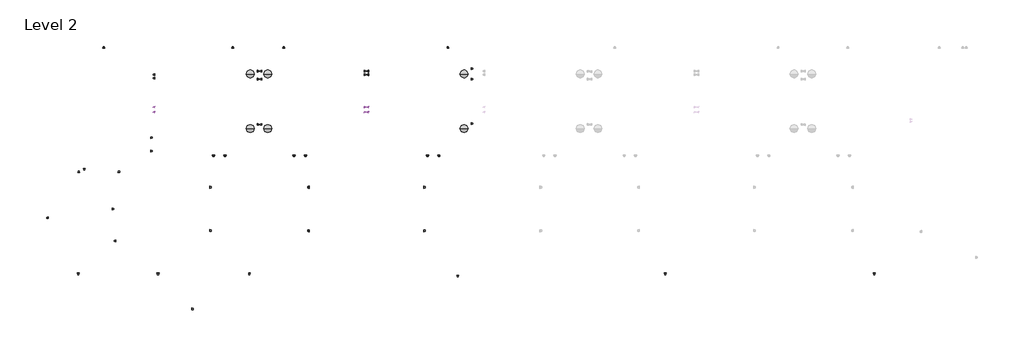
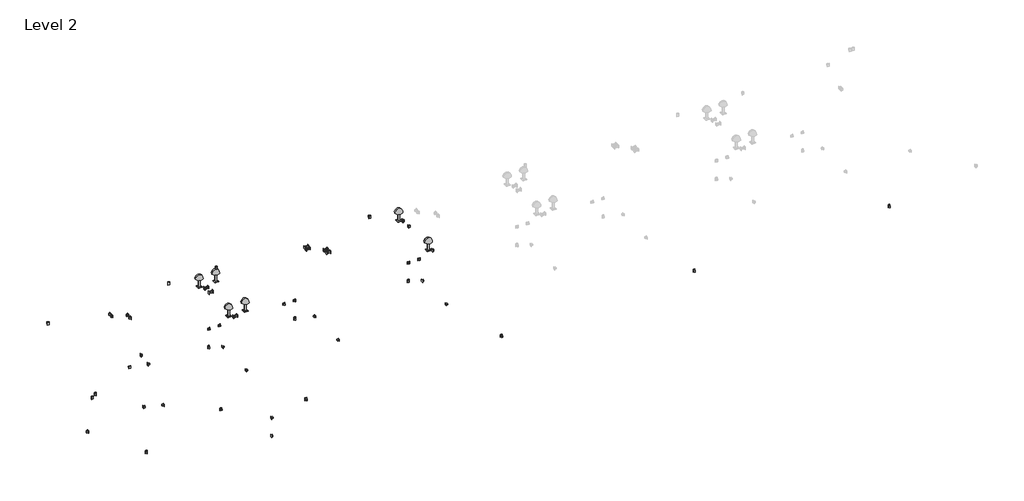
# One storey, part 1 of 2: 40 proxies, 16 switching devices, 6 light fixtures.
"""IFC4 building model written with IfcOpenShell, lengths in millimetres."""

import ifcopenshell
import ifcopenshell.guid

model = None  # the IFC model being written
_history = None  # IfcOwnerHistory: only IFC2X3 demands one
_inside = {}  # id of a spatial element -> (the spatial element, [elements in it])
_under = {}  # id of a project, library or spatial element -> (it, [spatial elements below it])
_declared = {}  # id of a project -> (the project, [libraries it declares])
_typed = {}  # id of a type object -> (the type object, [elements of that type])
_made_of = {}  # id of a material, layer set ... -> (it, [elements and type objects made of it])


def new_model(schema):
    """Start an empty IFC model of exactly this schema.

    Asked for "IFC4X3", IfcOpenShell would pick the latest addendum, in which some entities
    have other attributes; the version numbers below select the first issue.
    IFC2X3 requires an IfcOwnerHistory on every rooted entity: one is made here for all.
    """
    global model, _history
    if schema == "IFC4X3":
        model = ifcopenshell.file(schema_version=(4, 3, 0, 0))
    else:
        model = ifcopenshell.file(schema=schema)
    _inside.clear()
    _under.clear()
    _declared.clear()
    _typed.clear()
    _made_of.clear()
    _history = None
    if model.schema == "IFC2X3":
        org = make("IfcOrganization", Name="unknown")
        user = make(
            "IfcPersonAndOrganization",
            ThePerson=make("IfcPerson", FamilyName="unknown"),
            TheOrganization=org,
        )
        app = make(
            "IfcApplication",
            ApplicationDeveloper=org,
            Version="unknown",
            ApplicationFullName="unknown",
            ApplicationIdentifier="unknown",
        )
        _history = make(
            "IfcOwnerHistory",
            OwningUser=user,
            OwningApplication=app,
            ChangeAction="ADDED",
            CreationDate=0,
        )
    return model


def make(cls, **values):
    """One entity of the class cls with the attributes given. An attribute that is None is left unset."""
    return model.create_entity(
        cls, **{name: value for name, value in values.items() if value is not None}
    )


def rooted(cls, **values):
    """An entity with a GlobalId (a new one), such as an element, a storey or a relation."""
    return make(cls, GlobalId=ifcopenshell.guid.new(), OwnerHistory=_history, **values)


def si_unit(unit_type, name, prefix=None):
    """IfcSIUnit, for example si_unit("LENGTHUNIT", "METRE", prefix="MILLI")."""
    return make("IfcSIUnit", UnitType=unit_type, Prefix=prefix, Name=name)


def assignment(units):
    """IfcUnitAssignment: the units of a project."""
    return None if units is None else make("IfcUnitAssignment", Units=units)


def point(xyz):
    """IfcCartesianPoint."""
    return None if xyz is None else make("IfcCartesianPoint", Coordinates=xyz)


def direction(xyz):
    """IfcDirection."""
    return None if xyz is None else make("IfcDirection", DirectionRatios=xyz)


def frame(location, z_axis=None, x_axis=None):
    """IfcAxis2Placement3D, a coordinate frame: its origin and axes. An axis left out is left unset."""
    return make(
        "IfcAxis2Placement3D",
        Location=point(location),
        Axis=direction(z_axis),
        RefDirection=direction(x_axis),
    )


def frame_2d(location, x_axis=None):
    """IfcAxis2Placement2D, a coordinate frame in the plane: its origin and x axis."""
    return make(
        "IfcAxis2Placement2D", Location=point(location), RefDirection=direction(x_axis)
    )


def origin():
    """The frame at (0, 0, 0) with its axes left unset."""
    return frame((0.0, 0.0, 0.0))


def origin_with_axes():
    """The frame at (0, 0, 0) with the z axis (0, 0, 1) and the x axis (1, 0, 0) written out."""
    return frame((0.0, 0.0, 0.0), z_axis=(0.0, 0.0, 1.0), x_axis=(1.0, 0.0, 0.0))


def origin_2d():
    """The frame at (0, 0) in the plane with its x axis left unset."""
    return frame_2d((0.0, 0.0))


def place(relative_to, where):
    """IfcLocalPlacement: puts the frame where relative to a parent placement (None: the world)."""
    return make(
        "IfcLocalPlacement", PlacementRelTo=relative_to, RelativePlacement=where
    )


def context(
    kind, dimensions, precision=None, world=None, true_north=None, identifier=None
):
    """IfcGeometricRepresentationContext, for example the 3D "Model" context."""
    return make(
        "IfcGeometricRepresentationContext",
        ContextIdentifier=identifier,
        ContextType=kind,
        CoordinateSpaceDimension=dimensions,
        Precision=precision,
        WorldCoordinateSystem=world,
        TrueNorth=true_north,
    )


def project(units=None, contexts=None):
    """IfcProject with its units and contexts."""
    return rooted(
        "IfcProject",
        Name="project",
        RepresentationContexts=contexts,
        UnitsInContext=assignment(units),
    )


def spatial(cls, under=None, at=None, **own):
    """A site, building, storey or space (cls), placed at a placement, below another one or the project."""
    s = rooted(cls, ObjectPlacement=at, **own)
    if under is not None:
        _under.setdefault(under.id(), (under, []))[1].append(s)
    return s


def polyline(points):
    """IfcPolyline through the points."""
    return make("IfcPolyline", Points=[point(p) for p in points])


def circle_curve(where, radius):
    """IfcCircle in the frame where."""
    return make("IfcCircle", Position=where, Radius=radius)


def ellipse_curve(where, semi_axis1, semi_axis2):
    """IfcEllipse in the frame where."""
    return make(
        "IfcEllipse", Position=where, SemiAxis1=semi_axis1, SemiAxis2=semi_axis2
    )


def trimmed(basis, trim1, trim2, sense, master):
    """IfcTrimmedCurve: the piece of a basis curve between two trims."""
    return make(
        "IfcTrimmedCurve",
        BasisCurve=basis,
        Trim1=trim1,
        Trim2=trim2,
        SenseAgreement=sense,
        MasterRepresentation=master,
    )


def segment(curve, same_sense, transition):
    """IfcCompositeCurveSegment."""
    return make(
        "IfcCompositeCurveSegment",
        Transition=transition,
        SameSense=same_sense,
        ParentCurve=curve,
    )


def composite_curve(segments, self_intersect=None):
    """IfcCompositeCurve: segments joined end to end."""
    return make("IfcCompositeCurve", Segments=segments, SelfIntersect=self_intersect)


def outline(outer, holes=None, kind="AREA"):
    """IfcArbitraryClosedProfileDef: a profile drawn as a closed curve; with holes, ...WithVoids."""
    if holes is None:
        return make("IfcArbitraryClosedProfileDef", ProfileType=kind, OuterCurve=outer)
    return make(
        "IfcArbitraryProfileDefWithVoids",
        ProfileType=kind,
        OuterCurve=outer,
        InnerCurves=holes,
    )


def extrude(swept, where, along, depth):
    """IfcExtrudedAreaSolid: the profile swept, set in the frame where, extruded along a direction by depth."""
    return make(
        "IfcExtrudedAreaSolid",
        SweptArea=swept,
        Position=where,
        ExtrudedDirection=direction(along),
        Depth=depth,
    )


def shape(context_of_items, identifier, shape_type, items):
    """IfcShapeRepresentation: the items that make up one representation, for example the "Body"."""
    return make(
        "IfcShapeRepresentation",
        ContextOfItems=context_of_items,
        RepresentationIdentifier=identifier,
        RepresentationType=shape_type,
        Items=items,
    )


def source(mapping_origin, context_of_items, identifier, shape_type, items):
    """IfcRepresentationMap: a shape defined once, which mapped items show again and again."""
    return make(
        "IfcRepresentationMap",
        MappingOrigin=mapping_origin,
        MappedRepresentation=shape(context_of_items, identifier, shape_type, items),
    )


def transform(
    local_origin,
    x_axis=None,
    y_axis=None,
    z_axis=None,
    scale=None,
    scale2=None,
    scale3=None,
    uniform=True,
):
    """IfcCartesianTransformationOperator3D, or its non-uniform kind. x_axis, y_axis, z_axis: its Axis1, 2, 3."""
    if uniform:
        return make(
            "IfcCartesianTransformationOperator3D",
            Axis1=direction(x_axis),
            Axis2=direction(y_axis),
            LocalOrigin=point(local_origin),
            Scale=scale,
            Axis3=direction(z_axis),
        )
    return make(
        "IfcCartesianTransformationOperator3DnonUniform",
        Axis1=direction(x_axis),
        Axis2=direction(y_axis),
        LocalOrigin=point(local_origin),
        Scale=scale,
        Axis3=direction(z_axis),
        Scale2=scale2,
        Scale3=scale3,
    )


def mapped(mapping_source, mapping_target):
    """IfcMappedItem: shows the shape of a source again, moved by a transform."""
    return make(
        "IfcMappedItem", MappingSource=mapping_source, MappingTarget=mapping_target
    )


def made_of(thing, what):
    """Note that an element or type object is made of a material, layer set ...; save() writes the relation."""
    if what is not None:
        _made_of.setdefault(what.id(), (what, []))[1].append(thing)
    return thing


def element(
    cls,
    number,
    at=None,
    inside=None,
    cuts=None,
    type_object=None,
    material=None,
    context=None,
    identifier="Body",
    shape_type=None,
    held_by="IfcProductDefinitionShape",
    body=None,
    shapes=None,
    **own,
):
    """One element of the class cls, such as IfcWall. Its Tag is "e" and its number.

    at: its placement. inside: the storey or other place that contains it. cuts: it is an
    opening in that element (IfcRelVoidsElement). A single representation is given by context,
    identifier, shape_type and body (its items); several are given by shapes. held_by: the class
    of the entity that holds the representations. save() writes the other relations.
    """
    e = rooted(cls, Tag="e%d" % number, ObjectPlacement=at, **own)
    if body is not None:
        shapes = [shape(context, identifier, shape_type, body)]
    if shapes is not None:
        e.Representation = make(held_by, Representations=shapes)
    if inside is not None:
        _inside.setdefault(inside.id(), (inside, []))[1].append(e)
    if cuts is not None:
        rooted(
            "IfcRelVoidsElement", RelatingBuildingElement=cuts, RelatedOpeningElement=e
        )
    if type_object is not None:
        _typed.setdefault(type_object.id(), (type_object, []))[1].append(e)
    return made_of(e, material)


def aggregate(whole, parts):
    """IfcRelAggregates: a whole, such as a stair, and the parts it consists of."""
    return rooted("IfcRelAggregates", RelatingObject=whole, RelatedObjects=parts)


def save(model, path):
    """Write the relations noted so far, then the file.

    IfcRelAggregates (storeys below a building ...), IfcRelContainedInSpatialStructure (elements
    in a storey), IfcRelDefinesByType, IfcRelAssociatesMaterial and IfcRelDeclares: one each for
    every whole, place, type object, material and project.
    """
    for whole, parts in _under.values():
        aggregate(whole, parts)
    for where, things in _inside.values():
        rooted(
            "IfcRelContainedInSpatialStructure",
            RelatedElements=things,
            RelatingStructure=where,
        )
    for kind, things in _typed.values():
        rooted("IfcRelDefinesByType", RelatedObjects=things, RelatingType=kind)
    for what, things in _made_of.values():
        rooted("IfcRelAssociatesMaterial", RelatedObjects=things, RelatingMaterial=what)
    for by, libraries in _declared.values():
        rooted("IfcRelDeclares", RelatingContext=by, RelatedDefinitions=libraries)
    model.write(path)


def plane_surface(at):
    """IfcPlane: the flat surface through the origin of the frame at, square to its z axis."""
    return make("IfcPlane", Position=at)


def revolved_surface(curve, axis_point, axis_direction):
    """IfcSurfaceOfRevolution: the curve turned about the line through axis_point along axis_direction."""
    return make(
        "IfcSurfaceOfRevolution",
        SweptCurve=make("IfcArbitraryOpenProfileDef", ProfileType="CURVE", Curve=curve),
        AxisPosition=make("IfcAxis1Placement", Location=point(axis_point), Axis=direction(axis_direction)),
    )


def advanced_brep(points, edges, surfaces, faces):
    """IfcAdvancedBrep: a solid bounded by faces that lie on surfaces and meet in shared edges.

    An edge is (start, end): straight between two places in points (the first is 0);
    or (start, end, curve); or (start, end, curve, False) where it runs against its curve.
    A face is (place in surfaces, loops), or (place, loops, False) where it looks against
    its surface's normal. A loop lists edges by number (the first is 1), with a minus sign
    where the edge is run from its end to its start. The first loop is the outer one.
    """
    corners = [point(p) for p in points]
    vertices = [make("IfcVertexPoint", VertexGeometry=c) for c in corners]
    made = []
    for start, end, *more in edges:
        made.append(
            make(
                "IfcEdgeCurve",
                EdgeStart=vertices[start],
                EdgeEnd=vertices[end],
                EdgeGeometry=more[0] if more else make("IfcPolyline", Points=[corners[start], corners[end]]),
                SameSense=more[1] if len(more) > 1 else True,
            )
        )
    hull = []
    for where, loops, *sense in faces:
        bounds = []
        for j, loop in enumerate(loops):
            ring = [make("IfcOrientedEdge", EdgeElement=made[abs(k) - 1], Orientation=k > 0) for k in loop]
            bounds.append(
                make(
                    "IfcFaceOuterBound" if j == 0 else "IfcFaceBound",
                    Bound=make("IfcEdgeLoop", EdgeList=ring),
                    Orientation=True,
                )
            )
        hull.append(make("IfcAdvancedFace", Bounds=bounds, FaceSurface=surfaces[where], SameSense=sense[0] if sense else True))
    return make("IfcAdvancedBrep", Outer=make("IfcClosedShell", CfsFaces=hull))


def m_duplex_receptacle_top_switched_standard_10251bba(model_context):
    return source(origin(), model_context, "Body", "SweptSolid", [
        extrude(outline(polyline([(19.05, 38.1), (19.05, -38.1), (-19.05, -38.1), (-19.05, 38.1), (19.05, 38.1)])), frame((0.0, 0.0, -53.975), z_axis=(0.0, 0.0, 1.0), x_axis=(1.0, 0.0, 0.0)), (0.0, 0.0, 1.0), 53.975),
        extrude(outline(polyline([(34.925, 57.15), (34.925, -57.15), (-34.925, -57.15), (-34.925, 57.15), (34.925, 57.15)])), origin_with_axes(), (0.0, 0.0, 1.0), 4.7625),
    ])


def standard_8138c307(model_context):
    return source(origin(), model_context, "Body", "SweptSolid", [
        extrude(outline(polyline([(34.925, 57.15), (34.925, -57.15), (-34.925, -57.15), (-34.925, 57.15), (34.925, 57.15)]), holes=[composite_curve([segment(trimmed(circle_curve(frame_2d((0.6039572, -2.5749254)), 6.9441889), [point((-6.3402317, -2.5749254))], [point((7.5481461, -2.5749254))], True, "CARTESIAN"), True, "CONTINUOUS"), segment(trimmed(circle_curve(frame_2d((0.6039572, -2.5749254)), 6.9441889), [point((7.5481461, -2.5749254))], [point((-6.3402317, -2.5749254))], True, "CARTESIAN"), True, "CONTINUOUS")], self_intersect=False)]), origin_with_axes(), (0.0, 0.0, 1.0), 4.7625),
        extrude(outline(polyline([(19.05, 38.1), (19.05, -38.1), (-19.05, -38.1), (-19.05, 38.1), (19.05, 38.1)]), holes=[composite_curve([segment(trimmed(circle_curve(frame_2d((0.0, -0.79375)), 7.0675853), [point((-7.0675853, -0.79375))], [point((7.0675853, -0.79375))], True, "CARTESIAN"), True, "CONTINUOUS"), segment(trimmed(circle_curve(frame_2d((0.0, -0.79375)), 7.0675853), [point((7.0675853, -0.79375))], [point((-7.0675853, -0.79375))], True, "CARTESIAN"), True, "CONTINUOUS")], self_intersect=False)]), frame((0.0, 0.0, -53.975), z_axis=(0.0, 0.0, 1.0), x_axis=(1.0, 0.0, 0.0)), (0.0, 0.0, 1.0), 53.975),
    ])


def table_lamp_hemispheric_60w_230v_02721d88(model_context):
    return source(origin(), model_context, "Body", "SolidModel", [
        advanced_brep(
        [(0.0, 0.0, 524.5095504), (152.4, 0.0, 372.1095504), (-152.4, 0.0, 372.1095504), (-146.05, 0.0, 372.1095504), (146.05, 0.0, 372.1095504), (0.0, 0.0, 518.1595504)],
        [
            (0, 1, circle_curve(frame((0.0, 0.0, 372.1095504), z_axis=(0.0, 1.0, 0.0), x_axis=(1.0, 0.0, 0.0)), 152.4)),
            (1, 2, circle_curve(frame((0.0, 0.0, 372.1095504), z_axis=(0.0, 0.0, 1.0), x_axis=(1.0, 0.0, 0.0)), 152.4)),
            (2, 0, circle_curve(frame((0.0, 0.0, 372.1095504), z_axis=(0.0, 1.0, 0.0), x_axis=(-1.0, 0.0, 0.0)), 152.4)),
            (2, 1, circle_curve(frame((0.0, 0.0, 372.1095504), z_axis=(0.0, 0.0, 1.0), x_axis=(1.0, 0.0, 0.0)), 152.4)),
            (3, 4, circle_curve(frame((0.0, 0.0, 372.1095504), z_axis=(0.0, 0.0, -1.0), x_axis=(1.0, 0.0, 0.0)), 146.05)),
            (4, 5, circle_curve(frame((0.0, 0.0, 372.1095504), z_axis=(0.0, -1.0, 0.0), x_axis=(1.0, 0.0, 0.0)), 146.05)),
            (5, 3, circle_curve(frame((0.0, 0.0, 372.1095504), z_axis=(0.0, -1.0, 0.0), x_axis=(-1.0, 0.0, 0.0)), 146.05)),
            (4, 3, circle_curve(frame((0.0, 0.0, 372.1095504), z_axis=(0.0, 0.0, -1.0), x_axis=(1.0, 0.0, 0.0)), 146.05)),
            (1, 4),
            (3, 2),
        ],
        [
            revolved_surface(trimmed(ellipse_curve(frame((0.0, 0.0, 372.1095504), z_axis=(0.0, -1.0, 0.0), x_axis=(1.0, 0.0, 0.0)), 152.4, 152.4), [point((152.4, 0.0, 372.1095504))], [point((0.0, 0.0, 524.5095504))], True, "CARTESIAN"), (0.0, 0.0, 552.6321699), (0.0, 0.0, 1.0)),
            revolved_surface(trimmed(ellipse_curve(frame((0.0, 0.0, 372.1095504), z_axis=(0.0, 1.0, 0.0), x_axis=(1.0, 0.0, 0.0)), 146.05, 146.05), [point((0.0, 0.0, 518.1595504))], [point((146.05, 0.0, 372.1095504))], True, "CARTESIAN"), (0.0, 0.0, 552.6321699), (0.0, 0.0, 1.0)),
            plane_surface(frame((0.0, 0.0, 372.1095504), z_axis=(0.0, 0.0, -1.0), x_axis=(1.0, 0.0, 0.0))),
        ],
        [
            (0, [[1, 2, 3]]),
            (0, [[-3, 4, -1]]),
            (1, [[5, 6, 7]]),
            (1, [[8, -7, -6]]),
            (2, [[-2, 9, -5, 10]]),
            (2, [[-4, -10, -8, -9]]),
        ],
    ),
        extrude(outline(composite_curve([segment(trimmed(circle_curve(origin_2d(), 6.35), [point((-6.35, 0.0))], [point((6.35, 0.0))], False, "CARTESIAN"), True, "CONTINUOUS"), segment(trimmed(circle_curve(origin_2d(), 6.35), [point((6.35, 0.0))], [point((-6.35, 0.0))], False, "CARTESIAN"), True, "CONTINUOUS")], self_intersect=False)), frame((0.0, 0.0, 330.2), z_axis=(0.0, 0.0, 1.0), x_axis=(1.0, 0.0, 0.0)), (0.0, 0.0, 1.0), 63.5),
        extrude(outline(polyline([(25.4, -25.4), (-25.4, -25.4), (-25.4, 25.4), (25.4, 25.4), (25.4, -25.4)])), frame((0.0, 0.0, 25.4), z_axis=(0.0, 0.0, 1.0), x_axis=(1.0, 0.0, 0.0)), (0.0, 0.0, 1.0), 304.8),
        advanced_brep(
        [(-66.7336963, -50.8, 12.7), (-34.9836963, -50.8, 12.7), (-47.6836963, -50.8, 0.0), (-54.0336963, -50.8, 0.0), (-54.0336963, -50.8, 12.7), (-47.6836963, -50.8, 12.7)],
        [
            (0, 1, circle_curve(frame((-50.8586963, -50.8, 12.7), z_axis=(0.0, 0.0, -1.0), x_axis=(1.0, 0.0, 0.0)), 15.875)),
            (1, 2, circle_curve(frame((-47.6836963, -50.8, 12.7), z_axis=(0.0, 1.0, 0.0), x_axis=(1.0, 0.0, 0.0)), 12.7)),
            (2, 3, circle_curve(frame((-50.8586963, -50.8, 0.0), z_axis=(0.0, 0.0, 1.0), x_axis=(1.0, 0.0, 0.0)), 3.175)),
            (3, 0, circle_curve(frame((-54.0336963, -50.8, 12.7), z_axis=(0.0, 1.0, 0.0), x_axis=(-1.0, 0.0, 0.0)), 12.7)),
            (1, 0, circle_curve(frame((-50.8586963, -50.8, 12.7), z_axis=(0.0, 0.0, -1.0), x_axis=(1.0, 0.0, 0.0)), 15.875)),
            (3, 2, circle_curve(frame((-50.8586963, -50.8, 0.0), z_axis=(0.0, 0.0, 1.0), x_axis=(1.0, 0.0, 0.0)), 3.175)),
            (4, 5, circle_curve(frame((-50.8586963, -50.8, 12.7), z_axis=(0.0, 0.0, -1.0), x_axis=(1.0, 0.0, 0.0)), 3.175)),
            (5, 1),
            (0, 4),
            (5, 4, circle_curve(frame((-50.8586963, -50.8, 12.7), z_axis=(0.0, 0.0, -1.0), x_axis=(1.0, 0.0, 0.0)), 3.175)),
            (2, 5),
            (4, 3),
        ],
        [
            revolved_surface(trimmed(ellipse_curve(frame((-47.6836963, -50.8, 12.7), z_axis=(0.0, -1.0, 0.0), x_axis=(1.0, 0.0, 0.0)), 12.7, 12.7), [point((-47.6836963, -50.8, 0.0))], [point((-34.9836963, -50.8, 12.7))], True, "CARTESIAN"), (-50.8586963, -50.8, 36.0623287), (0.0, 0.0, 1.0)),
            plane_surface(frame((-50.8586963, -50.8, 12.7), z_axis=(0.0, 0.0, 1.0), x_axis=(1.0, 0.0, 0.0))),
            revolved_surface(polyline([(-47.6836963, -50.8, 12.7), (-47.6836963, -50.8, 0.0)]), (-50.8586963, -50.8, 36.0623287), (0.0, 0.0, 1.0)),
        ],
        [
            (0, [[1, 2, 3, 4]]),
            (0, [[5, -4, 6, -2]]),
            (1, [[7, 8, -1, 9]]),
            (1, [[10, -9, -5, -8]]),
            (2, [[-3, 11, -7, 12]]),
            (2, [[-6, -12, -10, -11]]),
        ],
    ),
        advanced_brep(
        [(-66.7581301, 50.8, 12.7), (-35.0081301, 50.8, 12.7), (-47.7081301, 50.8, 0.0), (-54.0581301, 50.8, 0.0), (-54.0581301, 50.8, 12.7), (-47.7081301, 50.8, 12.7)],
        [
            (0, 1, circle_curve(frame((-50.8831301, 50.8, 12.7), z_axis=(0.0, 0.0, -1.0), x_axis=(1.0, 0.0, 0.0)), 15.875)),
            (1, 2, circle_curve(frame((-47.7081301, 50.8, 12.7), z_axis=(0.0, 1.0, 0.0), x_axis=(1.0, 0.0, 0.0)), 12.7)),
            (2, 3, circle_curve(frame((-50.8831301, 50.8, 0.0), z_axis=(0.0, 0.0, 1.0), x_axis=(1.0, 0.0, 0.0)), 3.175)),
            (3, 0, circle_curve(frame((-54.0581301, 50.8, 12.7), z_axis=(0.0, 1.0, 0.0), x_axis=(-1.0, 0.0, 0.0)), 12.7)),
            (1, 0, circle_curve(frame((-50.8831301, 50.8, 12.7), z_axis=(0.0, 0.0, -1.0), x_axis=(1.0, 0.0, 0.0)), 15.875)),
            (3, 2, circle_curve(frame((-50.8831301, 50.8, 0.0), z_axis=(0.0, 0.0, 1.0), x_axis=(1.0, 0.0, 0.0)), 3.175)),
            (4, 5, circle_curve(frame((-50.8831301, 50.8, 12.7), z_axis=(0.0, 0.0, -1.0), x_axis=(1.0, 0.0, 0.0)), 3.175)),
            (5, 1),
            (0, 4),
            (5, 4, circle_curve(frame((-50.8831301, 50.8, 12.7), z_axis=(0.0, 0.0, -1.0), x_axis=(1.0, 0.0, 0.0)), 3.175)),
            (2, 5),
            (4, 3),
        ],
        [
            revolved_surface(trimmed(ellipse_curve(frame((-47.7081301, 50.8, 12.7), z_axis=(0.0, -1.0, 0.0), x_axis=(1.0, 0.0, 0.0)), 12.7, 12.7), [point((-47.7081301, 50.8, 0.0))], [point((-35.0081301, 50.8, 12.7))], True, "CARTESIAN"), (-50.8831301, 50.8, 36.0623287), (0.0, 0.0, 1.0)),
            plane_surface(frame((-50.8831301, 50.8, 12.7), z_axis=(0.0, 0.0, 1.0), x_axis=(1.0, 0.0, 0.0))),
            revolved_surface(polyline([(-47.708130100000005, 50.8, 12.7), (-47.708130100000005, 50.8, 0.0)]), (-50.8831301, 50.8, 36.0623287), (0.0, 0.0, 1.0)),
        ],
        [
            (0, [[1, 2, 3, 4]]),
            (0, [[5, -4, 6, -2]]),
            (1, [[7, 8, -1, 9]]),
            (1, [[10, -9, -5, -8]]),
            (2, [[-3, 11, -7, 12]]),
            (2, [[-6, -12, -10, -11]]),
        ],
    ),
        advanced_brep(
        [(34.9494337, -50.8, 12.7), (66.6994337, -50.8, 12.7), (53.9994337, -50.8, 0.0), (47.6494337, -50.8, 0.0), (47.6494337, -50.8, 12.7), (53.9994337, -50.8, 12.7)],
        [
            (0, 1, circle_curve(frame((50.8244337, -50.8, 12.7), z_axis=(0.0, 0.0, -1.0), x_axis=(1.0, 0.0, 0.0)), 15.875)),
            (1, 2, circle_curve(frame((53.9994337, -50.8, 12.7), z_axis=(0.0, 1.0, 0.0), x_axis=(1.0, 0.0, 0.0)), 12.7)),
            (2, 3, circle_curve(frame((50.8244337, -50.8, 0.0), z_axis=(0.0, 0.0, 1.0), x_axis=(1.0, 0.0, 0.0)), 3.175)),
            (3, 0, circle_curve(frame((47.6494337, -50.8, 12.7), z_axis=(0.0, 1.0, 0.0), x_axis=(-1.0, 0.0, 0.0)), 12.7)),
            (1, 0, circle_curve(frame((50.8244337, -50.8, 12.7), z_axis=(0.0, 0.0, -1.0), x_axis=(1.0, 0.0, 0.0)), 15.875)),
            (3, 2, circle_curve(frame((50.8244337, -50.8, 0.0), z_axis=(0.0, 0.0, 1.0), x_axis=(1.0, 0.0, 0.0)), 3.175)),
            (4, 5, circle_curve(frame((50.8244337, -50.8, 12.7), z_axis=(0.0, 0.0, -1.0), x_axis=(1.0, 0.0, 0.0)), 3.175)),
            (5, 1),
            (0, 4),
            (5, 4, circle_curve(frame((50.8244337, -50.8, 12.7), z_axis=(0.0, 0.0, -1.0), x_axis=(1.0, 0.0, 0.0)), 3.175)),
            (2, 5),
            (4, 3),
        ],
        [
            revolved_surface(trimmed(ellipse_curve(frame((53.9994337, -50.8, 12.7), z_axis=(0.0, -1.0, 0.0), x_axis=(1.0, 0.0, 0.0)), 12.7, 12.7), [point((53.9994337, -50.8, 0.0))], [point((66.6994337, -50.8, 12.7))], True, "CARTESIAN"), (50.8244337, -50.8, 36.0623287), (0.0, 0.0, 1.0)),
            plane_surface(frame((50.8244337, -50.8, 12.7), z_axis=(0.0, 0.0, 1.0), x_axis=(1.0, 0.0, 0.0))),
            revolved_surface(polyline([(53.9994337, -50.8, 12.7), (53.9994337, -50.8, 0.0)]), (50.8244337, -50.8, 36.0623287), (0.0, 0.0, 1.0)),
        ],
        [
            (0, [[1, 2, 3, 4]]),
            (0, [[5, -4, 6, -2]]),
            (1, [[7, 8, -1, 9]]),
            (1, [[10, -9, -5, -8]]),
            (2, [[-3, 11, -7, 12]]),
            (2, [[-6, -12, -10, -11]]),
        ],
    ),
        advanced_brep(
        [(34.925, 50.8, 12.7), (66.675, 50.8, 12.7), (53.975, 50.8, 0.0), (47.625, 50.8, 0.0), (47.625, 50.8, 12.7), (53.975, 50.8, 12.7)],
        [
            (0, 1, circle_curve(frame((50.8, 50.8, 12.7), z_axis=(0.0, 0.0, -1.0), x_axis=(1.0, 0.0, 0.0)), 15.875)),
            (1, 2, circle_curve(frame((53.975, 50.8, 12.7), z_axis=(0.0, 1.0, 0.0), x_axis=(1.0, 0.0, 0.0)), 12.7)),
            (2, 3, circle_curve(frame((50.8, 50.8, 0.0), z_axis=(0.0, 0.0, 1.0), x_axis=(1.0, 0.0, 0.0)), 3.175)),
            (3, 0, circle_curve(frame((47.625, 50.8, 12.7), z_axis=(0.0, 1.0, 0.0), x_axis=(-1.0, 0.0, 0.0)), 12.7)),
            (1, 0, circle_curve(frame((50.8, 50.8, 12.7), z_axis=(0.0, 0.0, -1.0), x_axis=(1.0, 0.0, 0.0)), 15.875)),
            (3, 2, circle_curve(frame((50.8, 50.8, 0.0), z_axis=(0.0, 0.0, 1.0), x_axis=(1.0, 0.0, 0.0)), 3.175)),
            (4, 5, circle_curve(frame((50.8, 50.8, 12.7), z_axis=(0.0, 0.0, -1.0), x_axis=(1.0, 0.0, 0.0)), 3.175)),
            (5, 1),
            (0, 4),
            (5, 4, circle_curve(frame((50.8, 50.8, 12.7), z_axis=(0.0, 0.0, -1.0), x_axis=(1.0, 0.0, 0.0)), 3.175)),
            (2, 5),
            (4, 3),
        ],
        [
            revolved_surface(trimmed(ellipse_curve(frame((53.975, 50.8, 12.7), z_axis=(0.0, -1.0, 0.0), x_axis=(1.0, 0.0, 0.0)), 12.7, 12.7), [point((53.975, 50.8, 0.0))], [point((66.675, 50.8, 12.7))], True, "CARTESIAN"), (50.8, 50.8, 36.0623287), (0.0, 0.0, 1.0)),
            plane_surface(frame((50.8, 50.8, 12.7), z_axis=(0.0, 0.0, 1.0), x_axis=(1.0, 0.0, 0.0))),
            revolved_surface(polyline([(53.974999999999994, 50.8, 12.7), (53.974999999999994, 50.8, 0.0)]), (50.8, 50.8, 36.0623287), (0.0, 0.0, 1.0)),
        ],
        [
            (0, [[1, 2, 3, 4]]),
            (0, [[5, -4, 6, -2]]),
            (1, [[7, 8, -1, 9]]),
            (1, [[10, -9, -5, -8]]),
            (2, [[-3, 11, -7, 12]]),
            (2, [[-6, -12, -10, -11]]),
        ],
    ),
        extrude(outline(polyline([(76.2, 76.2), (76.2, -76.2), (-76.2, -76.2), (-76.2, 76.2), (76.2, 76.2)])), frame((0.0, 0.0, 12.7), z_axis=(0.0, 0.0, 1.0), x_axis=(1.0, 0.0, 0.0)), (0.0, 0.0, 1.0), 12.7),
    ])


def lighting_switches_four_way_four_way_switch_ab144c04(model_context):
    return source(origin(), model_context, "Body", "SweptSolid", [
        extrude(outline(polyline([(43.0, -86.0), (-43.0, -86.0), (-43.0, 0.0), (43.0, 0.0), (43.0, -86.0)])), origin_with_axes(), (0.0, 0.0, 1.0), 5.0),
        extrude(outline(polyline([(27.0, -67.0), (-27.0, -67.0), (-27.0, -19.0), (27.0, -19.0), (27.0, -67.0)])), frame((0.0, 0.0, -54.0), z_axis=(0.0, 0.0, 1.0), x_axis=(1.0, 0.0, 0.0)), (0.0, 0.0, 1.0), 54.0),
    ])


model = new_model("IFC4")

# Units and contexts
model_context = context("Model", 3, world=origin())
ifc_project = project(units=[si_unit("LENGTHUNIT", "METRE", prefix="MILLI")], contexts=[model_context])

# Site, building, storey
site = spatial("IfcSite", under=ifc_project)
building = spatial("IfcBuilding", under=site)
storey = spatial("IfcBuildingStorey", under=building, Name="Level 2", Elevation=103800.0)

# Proxies
placement = place(None, origin())
m_duplex_receptacle_top_switched_standard_shape = m_duplex_receptacle_top_switched_standard_10251bba(model_context)
element("IfcBuildingElementProxy", 1, Name="M_Duplex Receptacle - Top Switched : Standard", ObjectType="M_Duplex Receptacle - Top Switched : Standard", at=placement, inside=storey, context=model_context, shape_type="MappedRepresentation", body=[
    mapped(m_duplex_receptacle_top_switched_standard_shape, transform((15910.005, 13930.039, 104190.0), x_axis=(0.0, -1.0, 0.0), y_axis=(0.0, 0.0, 1.0), z_axis=(-1.0, 0.0, 0.0))),
])
element("IfcBuildingElementProxy", 2, Name="M_Duplex Receptacle - Top Switched : Standard", ObjectType="M_Duplex Receptacle - Top Switched : Standard", at=placement, inside=storey, context=model_context, shape_type="MappedRepresentation", body=[
    mapped(m_duplex_receptacle_top_switched_standard_shape, transform((15910.005, 12275.0390001, 104190.0), x_axis=(0.0, -1.0, 0.0), y_axis=(0.0, 0.0, 1.0), z_axis=(-1.0, 0.0, 0.0))),
])
element("IfcBuildingElementProxy", 3, Name="M_Duplex Receptacle - Top Switched : Standard", ObjectType="M_Duplex Receptacle - Top Switched : Standard", at=placement, inside=storey, context=model_context, shape_type="MappedRepresentation", body=[
    mapped(m_duplex_receptacle_top_switched_standard_shape, transform((8101.5167855, 13930.039, 104190.0), x_axis=(0.0, 1.0, 0.0), y_axis=(0.0, 0.0, 1.0), z_axis=(1.0, 0.0, 0.0))),
])
element("IfcBuildingElementProxy", 4, Name="M_Duplex Receptacle - Top Switched : Standard", ObjectType="M_Duplex Receptacle - Top Switched : Standard", at=placement, inside=storey, context=model_context, shape_type="MappedRepresentation", body=[
    mapped(m_duplex_receptacle_top_switched_standard_shape, transform((8101.5167855, 12250.0390001, 104190.0), x_axis=(0.0, 1.0, 0.0), y_axis=(0.0, 0.0, 1.0), z_axis=(1.0, 0.0, 0.0))),
])
element("IfcBuildingElementProxy", 5, Name="M_Duplex Receptacle - Top Switched : Standard", ObjectType="M_Duplex Receptacle - Top Switched : Standard", at=placement, inside=storey, context=model_context, shape_type="MappedRepresentation", body=[
    mapped(m_duplex_receptacle_top_switched_standard_shape, transform((7951.5167855, 13930.039, 104190.0), x_axis=(0.0, -1.0, 0.0), y_axis=(0.0, 0.0, 1.0), z_axis=(-1.0, 0.0, 0.0))),
])
element("IfcBuildingElementProxy", 6, Name="M_Duplex Receptacle - Top Switched : Standard", ObjectType="M_Duplex Receptacle - Top Switched : Standard", at=placement, inside=storey, context=model_context, shape_type="MappedRepresentation", body=[
    mapped(m_duplex_receptacle_top_switched_standard_shape, transform((7951.5167855, 12250.0390001, 104190.0), x_axis=(0.0, -1.0, 0.0), y_axis=(0.0, 0.0, 1.0), z_axis=(-1.0, 0.0, 0.0))),
])
element("IfcBuildingElementProxy", 7, Name="M_Receptacle - 220V : Standard", ObjectType="M_Receptacle - 220V : Standard", at=placement, inside=storey, context=model_context, shape_type="MappedRepresentation", body=[
    mapped(m_duplex_receptacle_top_switched_standard_shape, transform((14267.9543134, 11096.4090428, 104190.0), x_axis=(-1.0, 0.0, 0.0), y_axis=(0.0, 0.0, 1.0), z_axis=(0.0, 1.0, 0.0))),
])
element("IfcBuildingElementProxy", 8, Name="M_Receptacle - 220V : Standard", ObjectType="M_Receptacle - 220V : Standard", at=placement, inside=storey, context=model_context, shape_type="MappedRepresentation", body=[
    mapped(m_duplex_receptacle_top_switched_standard_shape, transform((12081.5613786, 12710.0390001, 105212.0), x_axis=(0.0, 1.0, 0.0), y_axis=(0.0, 0.0, 1.0), z_axis=(1.0, 0.0, 0.0))),
])
element("IfcBuildingElementProxy", 9, Name="M_Receptacle - 220V : Standard", ObjectType="M_Receptacle - 220V : Standard", at=placement, inside=storey, context=model_context, shape_type="MappedRepresentation", body=[
    mapped(m_duplex_receptacle_top_switched_standard_shape, transform((12081.5613786, 14110.039, 104517.0), x_axis=(0.0, 1.0, 0.0), y_axis=(0.0, 0.0, 1.0), z_axis=(1.0, 0.0, 0.0))),
])
element("IfcBuildingElementProxy", 10, Name="M_Receptacle - 220V : Standard", ObjectType="M_Receptacle - 220V : Standard", at=placement, inside=storey, context=model_context, shape_type="MappedRepresentation", body=[
    mapped(m_duplex_receptacle_top_switched_standard_shape, transform((15040.005, 15100.039, 104190.0), x_axis=(1.0, 0.0, 0.0), y_axis=(0.0, 0.0, 1.0), z_axis=(0.0, -1.0, 0.0))),
])
element("IfcBuildingElementProxy", 11, Name="M_Receptacle - 220V : Standard", ObjectType="M_Receptacle - 220V : Standard", at=placement, inside=storey, context=model_context, shape_type="MappedRepresentation", body=[
    mapped(m_duplex_receptacle_top_switched_standard_shape, transform((8930.005, 15100.039, 104190.0), x_axis=(1.0, 0.0, 0.0), y_axis=(0.0, 0.0, 1.0), z_axis=(0.0, -1.0, 0.0))),
])
element("IfcBuildingElementProxy", 12, Name="M_Receptacle - 220V : Standard", ObjectType="M_Receptacle - 220V : Standard", at=placement, inside=storey, context=model_context, shape_type="MappedRepresentation", body=[
    mapped(m_duplex_receptacle_top_switched_standard_shape, transform((7030.005, 15100.039, 104190.0), x_axis=(1.0, 0.0, 0.0), y_axis=(0.0, 0.0, 1.0), z_axis=(0.0, -1.0, 0.0))),
])
element("IfcBuildingElementProxy", 13, Name="M_Receptacle - 220V : Standard", ObjectType="M_Receptacle - 220V : Standard", at=placement, inside=storey, context=model_context, shape_type="MappedRepresentation", body=[
    mapped(m_duplex_receptacle_top_switched_standard_shape, transform((9739.8253697, 11096.4090428, 104190.0), x_axis=(-1.0, 0.0, 0.0), y_axis=(0.0, 0.0, 1.0), z_axis=(0.0, 1.0, 0.0))),
])
element("IfcBuildingElementProxy", 14, Name="M_Receptacle - 220V : Standard", ObjectType="M_Receptacle - 220V : Standard", at=placement, inside=storey, context=model_context, shape_type="MappedRepresentation", body=[
    mapped(m_duplex_receptacle_top_switched_standard_shape, transform((6303.422276, 11096.4090428, 104190.0), x_axis=(-1.0, 0.0, 0.0), y_axis=(0.0, 0.0, 1.0), z_axis=(0.0, 1.0, 0.0))),
])
element("IfcBuildingElementProxy", 15, Name="M_Receptacle - 220V : Standard", ObjectType="M_Receptacle - 220V : Standard", at=placement, inside=storey, context=model_context, shape_type="MappedRepresentation", body=[
    mapped(m_duplex_receptacle_top_switched_standard_shape, transform((3973.5903641, 11250.0390001, 104190.0), x_axis=(0.0, -1.0, 0.0), y_axis=(0.0, 0.0, 1.0), z_axis=(-1.0, 0.0, 0.0))),
])
element("IfcBuildingElementProxy", 16, Name="M_Receptacle - 220V : Standard", ObjectType="M_Receptacle - 220V : Standard", at=placement, inside=storey, context=model_context, shape_type="MappedRepresentation", body=[
    mapped(m_duplex_receptacle_top_switched_standard_shape, transform((4123.5903641, 14105.0005078, 104520.0), x_axis=(0.0, 1.0, 0.0), y_axis=(0.0, 0.0, 1.0), z_axis=(1.0, 0.0, 0.0))),
])
element("IfcBuildingElementProxy", 17, Name="M_Receptacle - 220V : Standard", ObjectType="M_Receptacle - 220V : Standard", at=placement, inside=storey, context=model_context, shape_type="MappedRepresentation", body=[
    mapped(m_duplex_receptacle_top_switched_standard_shape, transform((4123.5903641, 12710.0390001, 105212.15), x_axis=(0.0, 1.0, 0.0), y_axis=(0.0, 0.0, 1.0), z_axis=(1.0, 0.0, 0.0))),
])
element("IfcBuildingElementProxy", 18, Name="M_Receptacle - 220V : Standard", ObjectType="M_Receptacle - 220V : Standard", at=placement, inside=storey, context=model_context, shape_type="MappedRepresentation", body=[
    mapped(m_duplex_receptacle_top_switched_standard_shape, transform((2220.005, 15100.039, 104190.0), x_axis=(1.0, 0.0, 0.0), y_axis=(0.0, 0.0, 1.0), z_axis=(0.0, -1.0, 0.0))),
])
element("IfcBuildingElementProxy", 19, Name="M_Receptacle - 220V : Standard", ObjectType="M_Receptacle - 220V : Standard", at=placement, inside=storey, context=model_context, shape_type="MappedRepresentation", body=[
    mapped(m_duplex_receptacle_top_switched_standard_shape, transform((1500.005, 10606.0701911, 104190.0), x_axis=(-1.0, 0.0, 0.0), y_axis=(0.0, 0.0, 1.0), z_axis=(0.0, 1.0, 0.0))),
])
element("IfcBuildingElementProxy", 20, Name="M_Receptacle - 220V : Standard", ObjectType="M_Receptacle - 220V : Standard", at=placement, inside=storey, context=model_context, shape_type="MappedRepresentation", body=[
    mapped(m_duplex_receptacle_top_switched_standard_shape, transform((1300.005, 10456.0701911, 104190.0), x_axis=(1.0, 0.0, 0.0), y_axis=(0.0, 0.0, 1.0), z_axis=(0.0, -1.0, 0.0))),
])
element("IfcBuildingElementProxy", 21, Name="M_Receptacle - 220V : Standard", ObjectType="M_Receptacle - 220V : Standard", at=placement, inside=storey, context=model_context, shape_type="MappedRepresentation", body=[
    mapped(m_duplex_receptacle_top_switched_standard_shape, transform((2548.0329505, 9090.0390001, 104190.0), x_axis=(0.0, -1.0, 0.0), y_axis=(0.0, 0.0, 1.0), z_axis=(-1.0, 0.0, 0.0))),
])
element("IfcBuildingElementProxy", 22, Name="M_Receptacle - 220V : Standard", ObjectType="M_Receptacle - 220V : Standard", at=placement, inside=storey, context=model_context, shape_type="MappedRepresentation", body=[
    mapped(m_duplex_receptacle_top_switched_standard_shape, transform((150.005, 8770.039, 104190.0), x_axis=(0.0, 1.0, 0.0), y_axis=(0.0, 0.0, 1.0), z_axis=(1.0, 0.0, 0.0))),
])
element("IfcBuildingElementProxy", 23, Name="M_Receptacle - 220V : Standard", ObjectType="M_Receptacle - 220V : Standard", at=placement, inside=storey, context=model_context, shape_type="MappedRepresentation", body=[
    mapped(m_duplex_receptacle_top_switched_standard_shape, transform((1280.005, 6700.039, 104190.0), x_axis=(-1.0, 0.0, 0.0), y_axis=(0.0, 0.0, 1.0), z_axis=(0.0, 1.0, 0.0))),
])
element("IfcBuildingElementProxy", 24, Name="M_Receptacle - 220V : Standard", ObjectType="M_Receptacle - 220V : Standard", at=placement, inside=storey, context=model_context, shape_type="MappedRepresentation", body=[
    mapped(m_duplex_receptacle_top_switched_standard_shape, transform((5500.0049999, 5370.0390001, 104190.0), x_axis=(0.0, -1.0, 0.0), y_axis=(0.0, 0.0, 1.0), z_axis=(-1.0, 0.0, 0.0))),
])
element("IfcBuildingElementProxy", 25, Name="M_Receptacle - 220V : Standard", ObjectType="M_Receptacle - 220V : Standard", at=placement, inside=storey, context=model_context, shape_type="MappedRepresentation", body=[
    mapped(m_duplex_receptacle_top_switched_standard_shape, transform((7650.005, 6700.039, 104190.0), x_axis=(-1.0, 0.0, 0.0), y_axis=(0.0, 0.0, 1.0), z_axis=(0.0, 1.0, 0.0))),
])
element("IfcBuildingElementProxy", 26, Name="M_Receptacle - 220V : Standard", ObjectType="M_Receptacle - 220V : Standard", at=placement, inside=storey, context=model_context, shape_type="MappedRepresentation", body=[
    mapped(m_duplex_receptacle_top_switched_standard_shape, transform((15400.005, 6625.039, 104190.0), x_axis=(-1.0, 0.0, 0.0), y_axis=(0.0, 0.0, 1.0), z_axis=(0.0, 1.0, 0.0))),
])
element("IfcBuildingElementProxy", 27, Name="M_Receptacle - 220V : Standard", ObjectType="M_Receptacle - 220V : Standard", at=placement, inside=storey, context=model_context, shape_type="MappedRepresentation", body=[
    mapped(m_duplex_receptacle_top_switched_standard_shape, transform((23126.2138022, 6700.039, 104190.0), x_axis=(-1.0, 0.0, 0.0), y_axis=(0.0, 0.0, 1.0), z_axis=(0.0, 1.0, 0.0))),
])
element("IfcBuildingElementProxy", 28, Name="M_Receptacle - 220V : Standard", ObjectType="M_Receptacle - 220V : Standard", at=placement, inside=storey, context=model_context, shape_type="MappedRepresentation", body=[
    mapped(m_duplex_receptacle_top_switched_standard_shape, transform((30910.005, 6700.039, 104190.0), x_axis=(-1.0, 0.0, 0.0), y_axis=(0.0, 0.0, 1.0), z_axis=(0.0, 1.0, 0.0))),
])
element("IfcBuildingElementProxy", 29, Name="M_Receptacle - 220V : Standard", ObjectType="M_Receptacle - 220V : Standard", at=placement, inside=storey, context=model_context, shape_type="MappedRepresentation", body=[
    mapped(m_duplex_receptacle_top_switched_standard_shape, transform((11931.5613786, 12710.0390001, 105212.0), x_axis=(0.0, -1.0, 0.0), y_axis=(0.0, 0.0, 1.0), z_axis=(-1.0, 0.0, 0.0))),
])
element("IfcBuildingElementProxy", 30, Name="M_Receptacle - 220V : Standard", ObjectType="M_Receptacle - 220V : Standard", at=placement, inside=storey, context=model_context, shape_type="MappedRepresentation", body=[
    mapped(m_duplex_receptacle_top_switched_standard_shape, transform((11931.5613786, 14110.039, 104520.0), x_axis=(0.0, -1.0, 0.0), y_axis=(0.0, 0.0, 1.0), z_axis=(-1.0, 0.0, 0.0))),
])
element("IfcBuildingElementProxy", 31, Name="M_Receptacle - DATA socket : Standard", ObjectType="M_Receptacle - DATA socket : Standard", at=placement, inside=storey, context=model_context, shape_type="MappedRepresentation", body=[
    mapped(m_duplex_receptacle_top_switched_standard_shape, transform((4123.5903641, 13976.0717391, 104520.0), x_axis=(0.0, 1.0, 0.0), y_axis=(0.0, 0.0, 1.0), z_axis=(1.0, 0.0, 0.0))),
])
element("IfcBuildingElementProxy", 32, Name="M_Receptacle - DATA socket : Standard", ObjectType="M_Receptacle - DATA socket : Standard", at=placement, inside=storey, context=model_context, shape_type="MappedRepresentation", body=[
    mapped(m_duplex_receptacle_top_switched_standard_shape, transform((3973.5903641, 11750.0390001, 104260.0), x_axis=(0.0, -1.0, 0.0), y_axis=(0.0, 0.0, 1.0), z_axis=(-1.0, 0.0, 0.0))),
])
element("IfcBuildingElementProxy", 33, Name="M_Receptacle - DATA socket : Standard", ObjectType="M_Receptacle - DATA socket : Standard", at=placement, inside=storey, context=model_context, shape_type="MappedRepresentation", body=[
    mapped(m_duplex_receptacle_top_switched_standard_shape, transform((7951.5167855, 14230.039, 104190.0), x_axis=(0.0, -1.0, 0.0), y_axis=(0.0, 0.0, 1.0), z_axis=(-1.0, 0.0, 0.0))),
])
element("IfcBuildingElementProxy", 34, Name="M_Receptacle - DATA socket : Standard", ObjectType="M_Receptacle - DATA socket : Standard", at=placement, inside=storey, context=model_context, shape_type="MappedRepresentation", body=[
    mapped(m_duplex_receptacle_top_switched_standard_shape, transform((11931.5613786, 14230.039, 104520.0), x_axis=(0.0, -1.0, 0.0), y_axis=(0.0, 0.0, 1.0), z_axis=(-1.0, 0.0, 0.0))),
])
element("IfcBuildingElementProxy", 35, Name="M_Receptacle - DATA socket : Standard", ObjectType="M_Receptacle - DATA socket : Standard", at=placement, inside=storey, context=model_context, shape_type="MappedRepresentation", body=[
    mapped(m_duplex_receptacle_top_switched_standard_shape, transform((12081.5613786, 14230.039, 104517.15), x_axis=(0.0, 1.0, 0.0), y_axis=(0.0, 0.0, 1.0), z_axis=(1.0, 0.0, 0.0))),
])
element("IfcBuildingElementProxy", 36, Name="M_Receptacle - DATA socket : Standard", ObjectType="M_Receptacle - DATA socket : Standard", at=placement, inside=storey, context=model_context, shape_type="MappedRepresentation", body=[
    mapped(m_duplex_receptacle_top_switched_standard_shape, transform((8101.5167855, 14230.039, 104190.0), x_axis=(0.0, 1.0, 0.0), y_axis=(0.0, 0.0, 1.0), z_axis=(1.0, 0.0, 0.0))),
])
element("IfcBuildingElementProxy", 37, Name="M_Receptacle - DATA socket : Standard", ObjectType="M_Receptacle - DATA socket : Standard", at=placement, inside=storey, context=model_context, shape_type="MappedRepresentation", body=[
    mapped(m_duplex_receptacle_top_switched_standard_shape, transform((15910.005, 14330.039, 104190.0), x_axis=(0.0, -1.0, 0.0), y_axis=(0.0, 0.0, 1.0), z_axis=(-1.0, 0.0, 0.0))),
])
standard_shape = standard_8138c307(model_context)
element("IfcBuildingElementProxy", 38, Name="M_Receptacle -TV /Satellite Socket : Standard", ObjectType="M_Receptacle -TV /Satellite Socket : Standard", at=placement, inside=storey, context=model_context, shape_type="MappedRepresentation", body=[
    mapped(standard_shape, transform((12081.5613786, 12890.0390001, 105212.0), x_axis=(0.0, 1.0, 0.0), y_axis=(0.0, 0.0, 1.0), z_axis=(1.0, 0.0, 0.0))),
])
element("IfcBuildingElementProxy", 39, Name="M_Receptacle -TV /Satellite Socket : Standard", ObjectType="M_Receptacle -TV /Satellite Socket : Standard", at=placement, inside=storey, context=model_context, shape_type="MappedRepresentation", body=[
    mapped(standard_shape, transform((4123.5903641, 12890.0390001, 105212.15), x_axis=(0.0, 1.0, 0.0), y_axis=(0.0, 0.0, 1.0), z_axis=(1.0, 0.0, 0.0))),
])
element("IfcBuildingElementProxy", 40, Name="M_Receptacle -TV /Satellite Socket : Standard", ObjectType="M_Receptacle -TV /Satellite Socket : Standard", at=placement, inside=storey, context=model_context, shape_type="MappedRepresentation", body=[
    mapped(standard_shape, transform((11931.5613786, 12890.0390001, 105212.0), x_axis=(0.0, -1.0, 0.0), y_axis=(0.0, 0.0, 1.0), z_axis=(-1.0, 0.0, 0.0))),
])

# Light fixtures
table_lamp_hemispheric_60w_230v_shape = table_lamp_hemispheric_60w_230v_02721d88(model_context)
element("IfcLightFixture", 41, ObjectType="Table Lamp - Hemispheric : 60W - 230V", at=placement, inside=storey, context=model_context, shape_type="MappedRepresentation", body=[
    mapped(table_lamp_hemispheric_60w_230v_shape, transform((15640.9293816, 12093.9035022, 104400.0), x_axis=(1.0, 0.0, 0.0), y_axis=(0.0, 1.0, 0.0), z_axis=(0.0, 0.0, 1.0))),
])
element("IfcLightFixture", 42, ObjectType="Table Lamp - Hemispheric : 60W - 230V", at=placement, inside=storey, context=model_context, shape_type="MappedRepresentation", body=[
    mapped(table_lamp_hemispheric_60w_230v_shape, transform((15640.9293816, 14131.1951689, 104400.0), x_axis=(1.0, 0.0, 0.0), y_axis=(0.0, 1.0, 0.0), z_axis=(0.0, 0.0, 1.0))),
])
element("IfcLightFixture", 43, ObjectType="Table Lamp - Hemispheric : 60W - 230V", at=placement, inside=storey, context=model_context, shape_type="MappedRepresentation", body=[
    mapped(table_lamp_hemispheric_60w_230v_shape, transform((8335.5554128, 12093.9035022, 104400.0), x_axis=(1.0, 0.0, 0.0), y_axis=(0.0, 1.0, 0.0), z_axis=(0.0, 0.0, 1.0))),
])
element("IfcLightFixture", 44, ObjectType="Table Lamp - Hemispheric : 60W - 230V", at=placement, inside=storey, context=model_context, shape_type="MappedRepresentation", body=[
    mapped(table_lamp_hemispheric_60w_230v_shape, transform((8335.5554128, 14131.1951689, 104400.0), x_axis=(1.0, 0.0, 0.0), y_axis=(0.0, 1.0, 0.0), z_axis=(0.0, 0.0, 1.0))),
])
element("IfcLightFixture", 45, ObjectType="Table Lamp - Hemispheric : 60W - 230V", at=placement, inside=storey, context=model_context, shape_type="MappedRepresentation", body=[
    mapped(table_lamp_hemispheric_60w_230v_shape, transform((7681.2861263, 12093.9035022, 104400.0), x_axis=(1.0, 0.0, 0.0), y_axis=(0.0, 1.0, 0.0), z_axis=(0.0, 0.0, 1.0))),
])
element("IfcLightFixture", 46, ObjectType="Table Lamp - Hemispheric : 60W - 230V", at=placement, inside=storey, context=model_context, shape_type="MappedRepresentation", body=[
    mapped(table_lamp_hemispheric_60w_230v_shape, transform((7681.2861263, 14131.1951689, 104400.0), x_axis=(1.0, 0.0, 0.0), y_axis=(0.0, 1.0, 0.0), z_axis=(0.0, 0.0, 1.0))),
])

# Switching devices
lighting_switches_four_way_four_way_switch_shape = lighting_switches_four_way_four_way_switch_ab144c04(model_context)
element("IfcSwitchingDevice", 47, ObjectType="Lighting Switches One Way : One Way Switch", at=placement, inside=storey, context=model_context, shape_type="MappedRepresentation", body=[
    mapped(lighting_switches_four_way_four_way_switch_shape, transform((2673.0329505, 7904.693557, 105000.0), x_axis=(0.0, 1.0, 0.0), y_axis=(0.0, 0.0, 1.0), z_axis=(1.0, 0.0, 0.0))),
])
element("IfcSwitchingDevice", 48, ObjectType="Lighting Switches One Way : One Way Switch", at=placement, inside=storey, context=model_context, shape_type="MappedRepresentation", body=[
    mapped(lighting_switches_four_way_four_way_switch_shape, transform((2787.036295, 10456.0701911, 105000.0), x_axis=(1.0, 0.0, 0.0), y_axis=(0.0, 0.0, 1.0), z_axis=(0.0, -1.0, 0.0))),
])
element("IfcSwitchingDevice", 49, ObjectType="Lighting Switches One Way : One Way Switch", at=placement, inside=storey, context=model_context, shape_type="MappedRepresentation", body=[
    mapped(lighting_switches_four_way_four_way_switch_shape, transform((6176.497276, 9910.5820743, 105000.0), x_axis=(0.0, -1.0, 0.0), y_axis=(0.0, 0.0, 1.0), z_axis=(-1.0, 0.0, 0.0))),
])
element("IfcSwitchingDevice", 50, ObjectType="Lighting Switches One Way : One Way Switch", at=placement, inside=storey, context=model_context, shape_type="MappedRepresentation", body=[
    mapped(lighting_switches_four_way_four_way_switch_shape, transform((14141.0293134, 9910.5820743, 105000.0), x_axis=(0.0, -1.0, 0.0), y_axis=(0.0, 0.0, 1.0), z_axis=(-1.0, 0.0, 0.0))),
])
element("IfcSwitchingDevice", 51, ObjectType="Lighting Switches One Way : One Way Switch", at=placement, inside=storey, context=model_context, shape_type="MappedRepresentation", body=[
    mapped(lighting_switches_four_way_four_way_switch_shape, transform((9866.7503697, 9911.1238803, 105000.0), x_axis=(0.0, 1.0, 0.0), y_axis=(0.0, 0.0, 1.0), z_axis=(1.0, 0.0, 0.0))),
])
element("IfcSwitchingDevice", 52, ObjectType="Lighting Switches One Way : One Way Switch", at=placement, inside=storey, context=model_context, shape_type="MappedRepresentation", body=[
    mapped(lighting_switches_four_way_four_way_switch_shape, transform((14699.0293134, 11096.4090428, 105000.0), x_axis=(-1.0, 0.0, 0.0), y_axis=(0.0, 0.0, 1.0), z_axis=(0.0, 1.0, 0.0))),
])
element("IfcSwitchingDevice", 53, ObjectType="Lighting Switches One Way : One Way Switch", at=placement, inside=storey, context=model_context, shape_type="MappedRepresentation", body=[
    mapped(lighting_switches_four_way_four_way_switch_shape, transform((14276.0293134, 11096.4090428, 105000.0), x_axis=(-1.0, 0.0, 0.0), y_axis=(0.0, 0.0, 1.0), z_axis=(0.0, 1.0, 0.0))),
])
element("IfcSwitchingDevice", 54, ObjectType="Lighting Switches One Way : One Way Switch", at=placement, inside=storey, context=model_context, shape_type="MappedRepresentation", body=[
    mapped(lighting_switches_four_way_four_way_switch_shape, transform((9308.7503697, 11096.4090428, 105000.0), x_axis=(-1.0, 0.0, 0.0), y_axis=(0.0, 0.0, 1.0), z_axis=(0.0, 1.0, 0.0))),
])
element("IfcSwitchingDevice", 55, ObjectType="Lighting Switches One Way : One Way Switch", at=placement, inside=storey, context=model_context, shape_type="MappedRepresentation", body=[
    mapped(lighting_switches_four_way_four_way_switch_shape, transform((6734.497276, 11096.4090428, 105000.0), x_axis=(-1.0, 0.0, 0.0), y_axis=(0.0, 0.0, 1.0), z_axis=(0.0, 1.0, 0.0))),
])
element("IfcSwitchingDevice", 56, ObjectType="Lighting Switches One Way : One Way Switch", at=placement, inside=storey, context=model_context, shape_type="MappedRepresentation", body=[
    mapped(lighting_switches_four_way_four_way_switch_shape, transform((6176.497276, 8294.4056984, 105000.0), x_axis=(0.0, -1.0, 0.0), y_axis=(0.0, 0.0, 1.0), z_axis=(-1.0, 0.0, 0.0))),
])
element("IfcSwitchingDevice", 57, ObjectType="Lighting Switches One Way : One Way Switch", at=placement, inside=storey, context=model_context, shape_type="MappedRepresentation", body=[
    mapped(lighting_switches_four_way_four_way_switch_shape, transform((9866.7503697, 8280.4056984, 105000.0), x_axis=(0.0, 1.0, 0.0), y_axis=(0.0, 0.0, 1.0), z_axis=(1.0, 0.0, 0.0))),
])
element("IfcSwitchingDevice", 58, ObjectType="Lighting Switches One Way : One Way Switch", at=placement, inside=storey, context=model_context, shape_type="MappedRepresentation", body=[
    mapped(lighting_switches_four_way_four_way_switch_shape, transform((14141.0293134, 8280.4056984, 105000.0), x_axis=(0.0, -1.0, 0.0), y_axis=(0.0, 0.0, 1.0), z_axis=(-1.0, 0.0, 0.0))),
])
element("IfcSwitchingDevice", 59, ObjectType="Lighting Switches One Way : One Way Switch", at=placement, inside=storey, context=model_context, shape_type="MappedRepresentation", body=[
    mapped(lighting_switches_four_way_four_way_switch_shape, transform((9731.7503697, 11096.4090428, 105000.0), x_axis=(-1.0, 0.0, 0.0), y_axis=(0.0, 0.0, 1.0), z_axis=(0.0, 1.0, 0.0))),
])
element("IfcSwitchingDevice", 60, ObjectType="Lighting Switches One Way : One Way Switch", at=placement, inside=storey, context=model_context, shape_type="MappedRepresentation", body=[
    mapped(lighting_switches_four_way_four_way_switch_shape, transform((6311.497276, 11096.4090428, 105000.0), x_axis=(-1.0, 0.0, 0.0), y_axis=(0.0, 0.0, 1.0), z_axis=(0.0, 1.0, 0.0))),
])
element("IfcSwitchingDevice", 61, ObjectType="Lighting Switches Two Way : Two Way Switch", at=placement, inside=storey, context=model_context, shape_type="MappedRepresentation", body=[
    mapped(lighting_switches_four_way_four_way_switch_shape, transform((4250.0050001, 6700.039, 105000.0), x_axis=(-1.0, 0.0, 0.0), y_axis=(0.0, 0.0, 1.0), z_axis=(0.0, 1.0, 0.0))),
])
element("IfcSwitchingDevice", 62, ObjectType="Lighting Switches Two Way : Two Way Switch", at=placement, inside=storey, context=model_context, shape_type="MappedRepresentation", body=[
    mapped(lighting_switches_four_way_four_way_switch_shape, transform((5500.0049999, 5370.0390001, 105000.0), x_axis=(0.0, -1.0, 0.0), y_axis=(0.0, 0.0, 1.0), z_axis=(-1.0, 0.0, 0.0))),
])

save(model, "model.ifc")

# Revit data of these elements
# Type "M_Duplex Receptacle - Top Switched : Standard"
#   Type Mark = "M_Duplex Receptacle - Top Switched"
#   Classification.OmniClass.21.Number = "21-04 50 30 50"
#   Classification.MasterFormat.Description = "Wiring Devices"
#   Classification.OmniClass.22.Number = "22-26 27 26"
#   Classification.OmniClass.21.Description = "Wiring Devices"
#   Classification.UniFormat.II.Description = "Wiring Devices"
#   Classification.MasterFormat.Number = "26 27 26"
#   Classification.OmniClass.23.Number = "23-35 27 11"
#   Classification.OmniClass.22.Description = "Wiring Devices"
#   Classification.OmniClass.23.Description = "Electrical Receptacles"
#   Classification.UniFormat.II.Number = "D5030.50"
#   COBie.Type.CreatedBy = "info@mma.ie"
#   COBie.Type.CreatedOn = "2017-07-25T10:15:16"
#   COBie.Type.Name = "M_Duplex Receptacle - Top Switched"
#   COBie.Type.Category = "23-35 27 11 : Electrical Receptacles"
#   COBie.Type.Description = "M_Duplex Receptacle - Top Switched_Standard"
#   COBie.Type.AssetType = "Fixed"
#   COBie.Type.Manufacturer = ""
#   COBie.Type.ModelNumber = ""
#   Keynote = "26 27 26.B"
#   COBie.Type.ReplacementCost = 0
#   Switch Voltage = 220 V
#   Recep.Width = 69.85 mm
#   Recep.Load = 180 VA
#   Recep.Height = 114.3 mm
#   Load = 180 VA
#   Default Elevation = 460 mm
#   COBie.Type = yes
#   Recep.Material = Stainless Steel
#   Load Classification = Receptacle
#   Assembly Code = ""
# Type "M_Receptacle - 220V : Standard"
#   Type Mark = "M_Receptacle - 220V"
#   Classification.OmniClass.21.Number = "21-04 50 30 50"
#   Classification.MasterFormat.Description = "Wiring Devices"
#   Classification.OmniClass.22.Number = "22-26 27 26"
#   Classification.OmniClass.21.Description = "Wiring Devices"
#   Classification.UniFormat.II.Description = "Wiring Devices"
#   Classification.MasterFormat.Number = "26 27 26"
#   Classification.OmniClass.23.Number = "23-35 27 11"
#   Classification.OmniClass.22.Description = "Wiring Devices"
#   Classification.OmniClass.23.Description = "Electrical Receptacles"
#   Classification.UniFormat.II.Number = "D5030.50"
#   COBie.Type.CreatedBy = "info@mma.ie"
#   COBie.Type.CreatedOn = "2017-07-25T10:15:16"
#   COBie.Type.Name = "M_Receptacle - 220V"
#   COBie.Type.Category = "23-35 27 11 : Electrical Receptacles"
#   COBie.Type.Description = "M_Receptacle - 220V_Standard"
#   COBie.Type.AssetType = "Fixed"
#   COBie.Type.Manufacturer = ""
#   COBie.Type.ModelNumber = ""
#   Keynote = "26 27 26.D"
#   COBie.Type.ReplacementCost = 0
#   Switch Voltage = 220 V
#   Recep.Width [instance default] = 69.85 mm
#   Recep.Load = 180 VA
#   Recep.Height [instance default] = 114.3 mm
#   Load = 180 VA
#   Default Elevation = 460 mm
#   COBie.Type = yes
#   Recep.Material = Stainless Steel
#   Load Classification = Receptacle
#   Assembly Code = ""
# Type "M_Receptacle - DATA socket : Standard"
#   Type Mark = "M_Receptacle - DATA socket"
#   Classification.OmniClass.21.Number = "21-04 50 30 50"
#   Classification.MasterFormat.Description = "Wiring Devices"
#   Classification.OmniClass.22.Number = "22-26 27 26"
#   Classification.OmniClass.21.Description = "Wiring Devices"
#   Classification.UniFormat.II.Description = "Wiring Devices"
#   Classification.MasterFormat.Number = "26 27 26"
#   Classification.OmniClass.23.Number = "23-35 27 11"
#   Classification.OmniClass.22.Description = "Wiring Devices"
#   Classification.OmniClass.23.Description = "Electrical Receptacles"
#   Classification.UniFormat.II.Number = "D5030.50"
#   COBie.Type.CreatedBy = "info@mma.ie"
#   COBie.Type.CreatedOn = "2017-07-25T10:15:16"
#   COBie.Type.Name = "M_Receptacle - DATA socket"
#   COBie.Type.Category = "23-35 27 11 : Electrical Receptacles"
#   COBie.Type.Description = "M_Receptacle - DATA socket_Standard"
#   COBie.Type.AssetType = "Fixed"
#   COBie.Type.Manufacturer = ""
#   COBie.Type.ModelNumber = ""
#   Keynote = "26 27 26.E"
#   COBie.Type.ReplacementCost = 0
#   Switch Voltage = 220 V
#   Recep.Width = 69.85 mm
#   Recep.Load = 180 VA
#   Recep.Height [instance default] = 114.3 mm
#   Load = 180 VA
#   Default Elevation = 460 mm
#   COBie.Type = yes
#   Recep.Material = Stainless Steel
#   Load Classification = Receptacle
#   Assembly Code = ""
# Type "M_Receptacle -TV /Satellite Socket : Standard"
#   Type Mark = "M_Receptacle -TV"
#   Classification.OmniClass.21.Number = "21-04 50 30 50"
#   Classification.MasterFormat.Description = "Wiring Devices"
#   Classification.OmniClass.22.Number = "22-26 27 26"
#   Classification.OmniClass.21.Description = "Wiring Devices"
#   Classification.UniFormat.II.Description = "Wiring Devices"
#   Classification.MasterFormat.Number = "26 27 26"
#   Classification.OmniClass.23.Number = "23-35 27 11"
#   Classification.OmniClass.22.Description = "Wiring Devices"
#   Classification.OmniClass.23.Description = "Electrical Receptacles"
#   Classification.UniFormat.II.Number = "D5030.50"
#   COBie.Type.CreatedBy = "info@mma.ie"
#   COBie.Type.CreatedOn = "2017-07-25T10:15:16"
#   COBie.Type.Name = "M_Receptacle -TV"
#   COBie.Type.Category = "23-35 27 11 : Electrical Receptacles"
#   COBie.Type.Description = "M_Receptacle -TV /Satellite Socket_Standard"
#   COBie.Type.AssetType = "Fixed"
#   COBie.Type.Manufacturer = ""
#   COBie.Type.ModelNumber = ""
#   Keynote = "26 27 26.A"
#   COBie.Type.ReplacementCost = 0
#   Switch Voltage = 220 V
#   Recep.Width = 69.85 mm
#   Recep.Load = 180 VA
#   Recep.Height = 114.3 mm
#   Load = 180 VA
#   Default Elevation = 460 mm
#   COBie.Type = yes
#   Recep.Material = Stainless Steel
#   Load Classification = Receptacle
#   Assembly Code = ""
# Type "Table Lamp - Hemispheric : 60W - 230V"
#   Type Mark = "Table Lamp - Hemispheric"
#   Classification.OmniClass.23.Number = "23-35 47 11"
#   Classification.OmniClass.23.Description = "Lighting Fixtures"
#   COBie.Type.CreatedBy = "info@mma.ie"
#   COBie.Type.CreatedOn = "2017-07-25T10:15:16"
#   COBie.Type.Name = "Table Lamp - Hemispheric"
#   COBie.Type.Category = "23-35 47 11 : Lighting Fixtures"
#   COBie.Type.Description = "Table Lamp - Hemispheric_60W - 230V"
#   COBie.Type.AssetType = "Movable"
#   COBie.Type.Manufacturer = ""
#   COBie.Type.ModelNumber = ""
#   Photometric Web File = "TLAE1A19.ies"
#   Keynote = "26 51 13.B"
#   Assembly Code = "D5020220"
#   Lamp = "A-19"
#   COBie.Type.ReplacementCost = 0
#   Wattage = 60 W
#   built-in parameter 1150110 = 1 (stored number, unit not read)
#   built-in parameter 1114217 = 1 (stored number, unit not read)
#   built-in parameter 1150109 = 1 (stored number, unit not read)
#   T.L. Tilt Angle = 90.00°
#   T.L. Efficacy = 14.25 lm/W
#   built-in parameter 1150113 = 1 (stored number, unit not read)
#   Tilt Angle = 90.00°
#   built-in parameter 1150115 = 1 (stored number, unit not read)
#   built-in parameter 1150105 = 68.0387 (stored number, unit not read)
#   built-in parameter 1150112 = 1 (stored number, unit not read)
#   built-in parameter 1150114 = 1 (stored number, unit not read)
#   built-in parameter 1150107 = 2800 (stored number, unit not read)
#   built-in parameter 1150106 = 0.680387 (stored number, unit not read)
#   built-in parameter 1150104 = 1.32387 (stored number, unit not read)
#   Ballast Voltage = 230 V
#   built-in parameter 1114218 = 1 (stored number, unit not read)
#   built-in parameter 1150133 = 10 (stored number, unit not read)
#   Lumens = 855 lm
#   Apparent Load = 60 VA
#   COBie.Type = yes
#   built-in parameter 1150134 = 4
